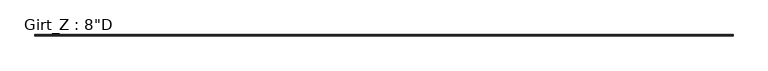
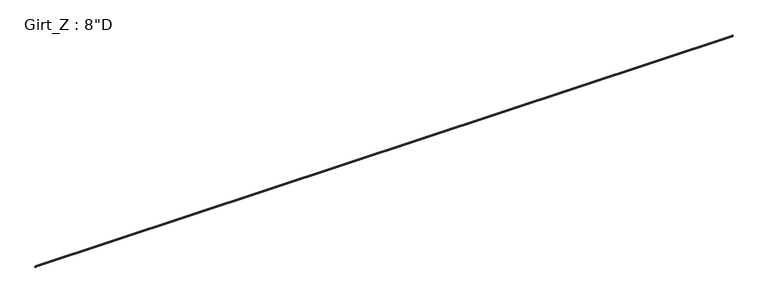
"""IFC4 building model written with IfcOpenShell, lengths in millimetres: beam geometry."""

import ifcopenshell
import ifcopenshell.guid

model = None  # the IFC model being written
_history = None  # IfcOwnerHistory: only IFC2X3 demands one
_inside = {}  # id of a spatial element -> (the spatial element, [elements in it])
_under = {}  # id of a project, library or spatial element -> (it, [spatial elements below it])
_declared = {}  # id of a project -> (the project, [libraries it declares])
_typed = {}  # id of a type object -> (the type object, [elements of that type])
_made_of = {}  # id of a material, layer set ... -> (it, [elements and type objects made of it])


def new_model(schema):
    """Start an empty IFC model of exactly this schema.

    Asked for "IFC4X3", IfcOpenShell would pick the latest addendum, in which some entities
    have other attributes; the version numbers below select the first issue.
    IFC2X3 requires an IfcOwnerHistory on every rooted entity: one is made here for all.
    """
    global model, _history
    if schema == "IFC4X3":
        model = ifcopenshell.file(schema_version=(4, 3, 0, 0))
    else:
        model = ifcopenshell.file(schema=schema)
    _inside.clear()
    _under.clear()
    _declared.clear()
    _typed.clear()
    _made_of.clear()
    _history = None
    if model.schema == "IFC2X3":
        org = make("IfcOrganization", Name="unknown")
        user = make(
            "IfcPersonAndOrganization",
            ThePerson=make("IfcPerson", FamilyName="unknown"),
            TheOrganization=org,
        )
        app = make(
            "IfcApplication",
            ApplicationDeveloper=org,
            Version="unknown",
            ApplicationFullName="unknown",
            ApplicationIdentifier="unknown",
        )
        _history = make(
            "IfcOwnerHistory",
            OwningUser=user,
            OwningApplication=app,
            ChangeAction="ADDED",
            CreationDate=0,
        )
    return model


def make(cls, **values):
    """One entity of the class cls with the attributes given. An attribute that is None is left unset."""
    return model.create_entity(
        cls, **{name: value for name, value in values.items() if value is not None}
    )


def rooted(cls, **values):
    """An entity with a GlobalId (a new one), such as an element, a storey or a relation."""
    return make(cls, GlobalId=ifcopenshell.guid.new(), OwnerHistory=_history, **values)


def si_unit(unit_type, name, prefix=None):
    """IfcSIUnit, for example si_unit("LENGTHUNIT", "METRE", prefix="MILLI")."""
    return make("IfcSIUnit", UnitType=unit_type, Prefix=prefix, Name=name)


def assignment(units):
    """IfcUnitAssignment: the units of a project."""
    return None if units is None else make("IfcUnitAssignment", Units=units)


def point(xyz):
    """IfcCartesianPoint."""
    return None if xyz is None else make("IfcCartesianPoint", Coordinates=xyz)


def direction(xyz):
    """IfcDirection."""
    return None if xyz is None else make("IfcDirection", DirectionRatios=xyz)


def frame(location, z_axis=None, x_axis=None):
    """IfcAxis2Placement3D, a coordinate frame: its origin and axes. An axis left out is left unset."""
    return make(
        "IfcAxis2Placement3D",
        Location=point(location),
        Axis=direction(z_axis),
        RefDirection=direction(x_axis),
    )


def frame_2d(location, x_axis=None):
    """IfcAxis2Placement2D, a coordinate frame in the plane: its origin and x axis."""
    return make(
        "IfcAxis2Placement2D", Location=point(location), RefDirection=direction(x_axis)
    )


def origin():
    """The frame at (0, 0, 0) with its axes left unset."""
    return frame((0.0, 0.0, 0.0))


def place(relative_to, where):
    """IfcLocalPlacement: puts the frame where relative to a parent placement (None: the world)."""
    return make(
        "IfcLocalPlacement", PlacementRelTo=relative_to, RelativePlacement=where
    )


def context(
    kind, dimensions, precision=None, world=None, true_north=None, identifier=None
):
    """IfcGeometricRepresentationContext, for example the 3D "Model" context."""
    return make(
        "IfcGeometricRepresentationContext",
        ContextIdentifier=identifier,
        ContextType=kind,
        CoordinateSpaceDimension=dimensions,
        Precision=precision,
        WorldCoordinateSystem=world,
        TrueNorth=true_north,
    )


def project(units=None, contexts=None):
    """IfcProject with its units and contexts."""
    return rooted(
        "IfcProject",
        Name="project",
        RepresentationContexts=contexts,
        UnitsInContext=assignment(units),
    )


def spatial(cls, under=None, at=None, **own):
    """A site, building, storey or space (cls), placed at a placement, below another one or the project."""
    s = rooted(cls, ObjectPlacement=at, **own)
    if under is not None:
        _under.setdefault(under.id(), (under, []))[1].append(s)
    return s


def polyline(points):
    """IfcPolyline through the points."""
    return make("IfcPolyline", Points=[point(p) for p in points])


def circle_curve(where, radius):
    """IfcCircle in the frame where."""
    return make("IfcCircle", Position=where, Radius=radius)


def trimmed(basis, trim1, trim2, sense, master):
    """IfcTrimmedCurve: the piece of a basis curve between two trims."""
    return make(
        "IfcTrimmedCurve",
        BasisCurve=basis,
        Trim1=trim1,
        Trim2=trim2,
        SenseAgreement=sense,
        MasterRepresentation=master,
    )


def segment(curve, same_sense, transition):
    """IfcCompositeCurveSegment."""
    return make(
        "IfcCompositeCurveSegment",
        Transition=transition,
        SameSense=same_sense,
        ParentCurve=curve,
    )


def composite_curve(segments, self_intersect=None):
    """IfcCompositeCurve: segments joined end to end."""
    return make("IfcCompositeCurve", Segments=segments, SelfIntersect=self_intersect)


def outline(outer, holes=None, kind="AREA"):
    """IfcArbitraryClosedProfileDef: a profile drawn as a closed curve; with holes, ...WithVoids."""
    if holes is None:
        return make("IfcArbitraryClosedProfileDef", ProfileType=kind, OuterCurve=outer)
    return make(
        "IfcArbitraryProfileDefWithVoids",
        ProfileType=kind,
        OuterCurve=outer,
        InnerCurves=holes,
    )


def extrude(swept, where, along, depth):
    """IfcExtrudedAreaSolid: the profile swept, set in the frame where, extruded along a direction by depth."""
    return make(
        "IfcExtrudedAreaSolid",
        SweptArea=swept,
        Position=where,
        ExtrudedDirection=direction(along),
        Depth=depth,
    )


def shape(context_of_items, identifier, shape_type, items):
    """IfcShapeRepresentation: the items that make up one representation, for example the "Body"."""
    return make(
        "IfcShapeRepresentation",
        ContextOfItems=context_of_items,
        RepresentationIdentifier=identifier,
        RepresentationType=shape_type,
        Items=items,
    )


def source(mapping_origin, context_of_items, identifier, shape_type, items):
    """IfcRepresentationMap: a shape defined once, which mapped items show again and again."""
    return make(
        "IfcRepresentationMap",
        MappingOrigin=mapping_origin,
        MappedRepresentation=shape(context_of_items, identifier, shape_type, items),
    )


def transform(
    local_origin,
    x_axis=None,
    y_axis=None,
    z_axis=None,
    scale=None,
    scale2=None,
    scale3=None,
    uniform=True,
):
    """IfcCartesianTransformationOperator3D, or its non-uniform kind. x_axis, y_axis, z_axis: its Axis1, 2, 3."""
    if uniform:
        return make(
            "IfcCartesianTransformationOperator3D",
            Axis1=direction(x_axis),
            Axis2=direction(y_axis),
            LocalOrigin=point(local_origin),
            Scale=scale,
            Axis3=direction(z_axis),
        )
    return make(
        "IfcCartesianTransformationOperator3DnonUniform",
        Axis1=direction(x_axis),
        Axis2=direction(y_axis),
        LocalOrigin=point(local_origin),
        Scale=scale,
        Axis3=direction(z_axis),
        Scale2=scale2,
        Scale3=scale3,
    )


def mapped(mapping_source, mapping_target):
    """IfcMappedItem: shows the shape of a source again, moved by a transform."""
    return make(
        "IfcMappedItem", MappingSource=mapping_source, MappingTarget=mapping_target
    )


def made_of(thing, what):
    """Note that an element or type object is made of a material, layer set ...; save() writes the relation."""
    if what is not None:
        _made_of.setdefault(what.id(), (what, []))[1].append(thing)
    return thing


def element(
    cls,
    number,
    at=None,
    inside=None,
    cuts=None,
    type_object=None,
    material=None,
    context=None,
    identifier="Body",
    shape_type=None,
    held_by="IfcProductDefinitionShape",
    body=None,
    shapes=None,
    **own,
):
    """One element of the class cls, such as IfcWall. Its Tag is "e" and its number.

    at: its placement. inside: the storey or other place that contains it. cuts: it is an
    opening in that element (IfcRelVoidsElement). A single representation is given by context,
    identifier, shape_type and body (its items); several are given by shapes. held_by: the class
    of the entity that holds the representations. save() writes the other relations.
    """
    e = rooted(cls, Tag="e%d" % number, ObjectPlacement=at, **own)
    if body is not None:
        shapes = [shape(context, identifier, shape_type, body)]
    if shapes is not None:
        e.Representation = make(held_by, Representations=shapes)
    if inside is not None:
        _inside.setdefault(inside.id(), (inside, []))[1].append(e)
    if cuts is not None:
        rooted(
            "IfcRelVoidsElement", RelatingBuildingElement=cuts, RelatedOpeningElement=e
        )
    if type_object is not None:
        _typed.setdefault(type_object.id(), (type_object, []))[1].append(e)
    return made_of(e, material)


def aggregate(whole, parts):
    """IfcRelAggregates: a whole, such as a stair, and the parts it consists of."""
    return rooted("IfcRelAggregates", RelatingObject=whole, RelatedObjects=parts)


def save(model, path):
    """Write the relations noted so far, then the file.

    IfcRelAggregates (storeys below a building ...), IfcRelContainedInSpatialStructure (elements
    in a storey), IfcRelDefinesByType, IfcRelAssociatesMaterial and IfcRelDeclares: one each for
    every whole, place, type object, material and project.
    """
    for whole, parts in _under.values():
        aggregate(whole, parts)
    for where, things in _inside.values():
        rooted(
            "IfcRelContainedInSpatialStructure",
            RelatedElements=things,
            RelatingStructure=where,
        )
    for kind, things in _typed.values():
        rooted("IfcRelDefinesByType", RelatedObjects=things, RelatingType=kind)
    for what, things in _made_of.values():
        rooted("IfcRelAssociatesMaterial", RelatedObjects=things, RelatingMaterial=what)
    for by, libraries in _declared.values():
        rooted("IfcRelDeclares", RelatingContext=by, RelatedDefinitions=libraries)
    model.write(path)


def beam_ab3afc21(model_context):
    return source(origin(), model_context, "Body", "SweptSolid", [
        extrude(outline(composite_curve([segment(polyline([(-63.5, 101.6), (-3.3734375, 101.6)]), True, "CONTINUOUS"), segment(trimmed(circle_curve(frame_2d((-3.3734375, 96.8375)), 4.7625), [point((-3.3734375, 101.6))], [point((1.3890625, 96.8375))], False, "CARTESIAN"), True, "CONTINUOUS"), segment(polyline([(1.3890625, 96.8375), (1.3890625, -96.8389339)]), True, "CONTINUOUS"), segment(trimmed(circle_curve(frame_2d((3.3748024, -96.8389339)), 1.9857399), [point((1.3890625, -96.8389339))], [point((3.2694106, -98.821875))], True, "CARTESIAN"), True, "CONTINUOUS"), segment(polyline([(3.2694106, -98.821875), (62.204539, -98.821875), (73.6169367, -85.221109), (75.745104, -87.0068534), (63.5, -101.6), (3.3734375, -101.6)]), True, "CONTINUOUS"), segment(trimmed(circle_curve(frame_2d((3.3734375, -96.8375)), 4.7625), [point((3.3734375, -101.6))], [point((-1.3890625, -96.8375))], False, "CARTESIAN"), True, "CONTINUOUS"), segment(polyline([(-1.3890625, -96.8375), (-1.3890625, 96.8381931)]), True, "CONTINUOUS"), segment(trimmed(circle_curve(frame_2d((-3.3741066, 96.8381931)), 1.9850441), [point((-1.3890625, 96.8381931))], [point((-3.3005807, 98.821875))], True, "CARTESIAN"), True, "CONTINUOUS"), segment(polyline([(-3.3005807, 98.821875), (-62.204539, 98.821875), (-73.6169367, 85.221109), (-75.745104, 87.0068534), (-63.5, 101.6)]), True, "CONTINUOUS")], self_intersect=False)), frame((-40605.744726, 0.0, 0.0), z_axis=(1.0, 0.0, 0.0), x_axis=(0.0, 1.0, 0.0)), (0.0, 0.0, 1.0), 80755.8769525),
    ])


if __name__ == "__main__":
    model = new_model("IFC4")
    model_context = context("Model", 3, world=origin())
    ifc_project = project(units=[si_unit("LENGTHUNIT", "METRE", prefix="MILLI")], contexts=[model_context])
    site = spatial("IfcSite", under=ifc_project)
    building = spatial("IfcBuilding", under=site)
    placement = place(None, origin())
    beam_shape = beam_ab3afc21(model_context)
    element("IfcBeam", 1, ObjectType="Girt_Z : 8\"D", at=placement, inside=building, context=model_context, shape_type="MappedRepresentation", body=[
        mapped(beam_shape, transform((0.0, 0.0, 0.0), x_axis=(1.0, 0.0, 0.0), y_axis=(0.0, 1.0, 0.0), z_axis=(0.0, 0.0, 1.0))),
    ])
    save(model, "model.ifc")

# Revit data of these elements
# Type "Girt_Z : 8\"D"
#   Web_Thickness = 0' - 0 7/64"
#   Length [instance default] = 10' - 0"
#   Leg_1 = 0' - 2 1/2"
#   Height = 0' - 8"
#   Structural Material [instance default] = none
# Element 1 (IfcBeam, "Girt_Z : 8\"D")
#   Structural Material = Steel
#   Materials on its faces: "Steel"
# Materials
#   "Steel": class "Metal", colour RGB 118 118 114, transparency 0, Description = "Steel, mill finish", Cost = 0
